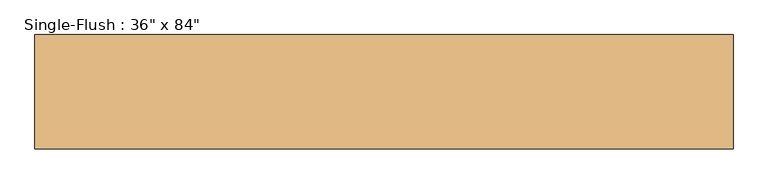
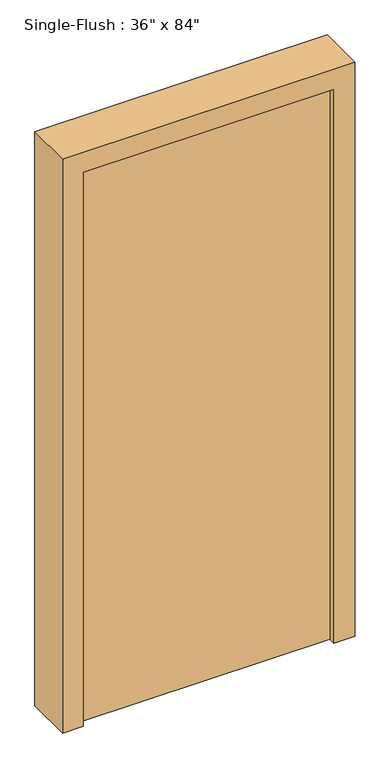
"""IFC4 building model written with IfcOpenShell, lengths in millimetres: door geometry."""

from ifc_helpers import new_model, si_unit, frame, origin, origin_with_axes, place, context, project, spatial, polyline, outline, extrude, source, transform, mapped, element, save


def door_c7c5887f(model_context):
    return source(origin(), model_context, "Body", "SweptSolid", [
        extrude(outline(polyline([(2209.8, 533.4), (2209.8, -533.4), (0.0, -533.4), (0.0, -457.2), (2133.6, -457.2), (2133.6, 457.2), (0.0, 457.2), (0.0, 533.4), (2209.8, 533.4)])), frame((0.0, -87.3125, 0.0), z_axis=(0.0, 1.0, 0.0), x_axis=(0.0, 0.0, 1.0)), (0.0, 0.0, 1.0), 174.625),
        extrude(outline(polyline([(457.2, -11.1125), (457.2, -61.9125), (-457.2, -61.9125), (-457.2, -11.1125), (457.2, -11.1125)])), origin_with_axes(), (0.0, 0.0, 1.0), 2133.6),
    ])


if __name__ == "__main__":
    model = new_model("IFC4")
    model_context = context("Model", 3, world=origin())
    ifc_project = project(units=[si_unit("LENGTHUNIT", "METRE", prefix="MILLI")], contexts=[model_context])
    site = spatial("IfcSite", under=ifc_project)
    building = spatial("IfcBuilding", under=site)
    placement = place(None, origin())
    door_shape = door_c7c5887f(model_context)
    element("IfcDoor", 1, ObjectType="Single-Flush : 36\" x 84\"", at=placement, inside=building, context=model_context, shape_type="MappedRepresentation", body=[
        mapped(door_shape, transform((0.0, 0.0, 0.0), x_axis=(1.0, 0.0, 0.0), y_axis=(0.0, 1.0, 0.0), z_axis=(0.0, 0.0, 1.0))),
    ])
    save(model, "model.ifc")

# Revit data of these elements
# Type "Single-Flush : 36\" x 84\""
#   Type Mark = "40"
#   Construction Type Id = "MDOOR"
#   Assembly Code = "C1020"
#   Analytic Construction = "Metal"
#   Thickness = 0' - 2"
#   Thermal Resistance (R) = 0.270117 (m²·K)/W
#   Heat Transfer Coefficient (U) = 3.7021 W/(m²·K)
#   Height = 7' - 0"
#   Trim Projection Ext = 0' - 1"
#   Trim Projection Int = 0' - 1"
#   Trim Width = 0' - 3"
#   Width = 3' - 0"
#   Door Material = Door - Panel
#   Frame Material = Door - Frame
#   Visual Light Transmittance = 0
#   Solar Heat Gain Coefficient = 0
#   Function = (empty or 0)
#   Wall Closure = (empty or 0)
# Element 1 (IfcDoor, "Single-Flush : 36\" x 84\"")
#   Materials on its faces: "Door - Frame", "Door - Panel"
# Materials
#   "Door - Panel": class "Wood", colour RGB 212 179 113, transparency 0, Cost = 0
#   "Door - Frame": class "Miscellaneous", colour RGB 65 65 65, transparency 0, Cost = 0
